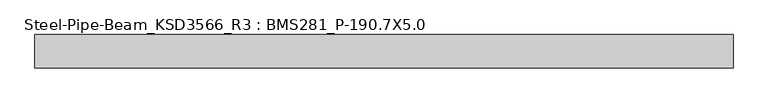
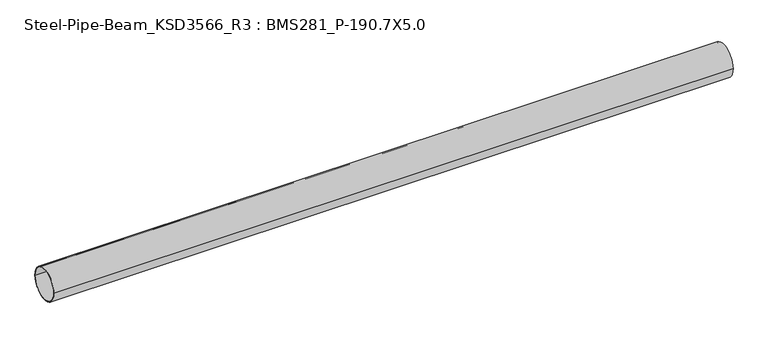
"""IFC4 building model written with IfcOpenShell, lengths in millimetres: member geometry, Steel-Pipe-Beam_KSD3566_R3 : BMS281_P-190.7X5.0."""

import ifcopenshell
import ifcopenshell.guid

model = None  # the IFC model being written
_history = None  # IfcOwnerHistory: only IFC2X3 demands one
_inside = {}  # id of a spatial element -> (the spatial element, [elements in it])
_under = {}  # id of a project, library or spatial element -> (it, [spatial elements below it])
_declared = {}  # id of a project -> (the project, [libraries it declares])
_typed = {}  # id of a type object -> (the type object, [elements of that type])
_made_of = {}  # id of a material, layer set ... -> (it, [elements and type objects made of it])


def new_model(schema):
    """Start an empty IFC model of exactly this schema.

    Asked for "IFC4X3", IfcOpenShell would pick the latest addendum, in which some entities
    have other attributes; the version numbers below select the first issue.
    IFC2X3 requires an IfcOwnerHistory on every rooted entity: one is made here for all.
    """
    global model, _history
    if schema == "IFC4X3":
        model = ifcopenshell.file(schema_version=(4, 3, 0, 0))
    else:
        model = ifcopenshell.file(schema=schema)
    _inside.clear()
    _under.clear()
    _declared.clear()
    _typed.clear()
    _made_of.clear()
    _history = None
    if model.schema == "IFC2X3":
        org = make("IfcOrganization", Name="unknown")
        user = make(
            "IfcPersonAndOrganization",
            ThePerson=make("IfcPerson", FamilyName="unknown"),
            TheOrganization=org,
        )
        app = make(
            "IfcApplication",
            ApplicationDeveloper=org,
            Version="unknown",
            ApplicationFullName="unknown",
            ApplicationIdentifier="unknown",
        )
        _history = make(
            "IfcOwnerHistory",
            OwningUser=user,
            OwningApplication=app,
            ChangeAction="ADDED",
            CreationDate=0,
        )
    return model


def make(cls, **values):
    """One entity of the class cls with the attributes given. An attribute that is None is left unset."""
    return model.create_entity(
        cls, **{name: value for name, value in values.items() if value is not None}
    )


def rooted(cls, **values):
    """An entity with a GlobalId (a new one), such as an element, a storey or a relation."""
    return make(cls, GlobalId=ifcopenshell.guid.new(), OwnerHistory=_history, **values)


def si_unit(unit_type, name, prefix=None):
    """IfcSIUnit, for example si_unit("LENGTHUNIT", "METRE", prefix="MILLI")."""
    return make("IfcSIUnit", UnitType=unit_type, Prefix=prefix, Name=name)


def assignment(units):
    """IfcUnitAssignment: the units of a project."""
    return None if units is None else make("IfcUnitAssignment", Units=units)


def point(xyz):
    """IfcCartesianPoint."""
    return None if xyz is None else make("IfcCartesianPoint", Coordinates=xyz)


def direction(xyz):
    """IfcDirection."""
    return None if xyz is None else make("IfcDirection", DirectionRatios=xyz)


def frame(location, z_axis=None, x_axis=None):
    """IfcAxis2Placement3D, a coordinate frame: its origin and axes. An axis left out is left unset."""
    return make(
        "IfcAxis2Placement3D",
        Location=point(location),
        Axis=direction(z_axis),
        RefDirection=direction(x_axis),
    )


def frame_2d(location, x_axis=None):
    """IfcAxis2Placement2D, a coordinate frame in the plane: its origin and x axis."""
    return make(
        "IfcAxis2Placement2D", Location=point(location), RefDirection=direction(x_axis)
    )


def origin():
    """The frame at (0, 0, 0) with its axes left unset."""
    return frame((0.0, 0.0, 0.0))


def origin_2d():
    """The frame at (0, 0) in the plane with its x axis left unset."""
    return frame_2d((0.0, 0.0))


def place(relative_to, where):
    """IfcLocalPlacement: puts the frame where relative to a parent placement (None: the world)."""
    return make(
        "IfcLocalPlacement", PlacementRelTo=relative_to, RelativePlacement=where
    )


def context(
    kind, dimensions, precision=None, world=None, true_north=None, identifier=None
):
    """IfcGeometricRepresentationContext, for example the 3D "Model" context."""
    return make(
        "IfcGeometricRepresentationContext",
        ContextIdentifier=identifier,
        ContextType=kind,
        CoordinateSpaceDimension=dimensions,
        Precision=precision,
        WorldCoordinateSystem=world,
        TrueNorth=true_north,
    )


def project(units=None, contexts=None):
    """IfcProject with its units and contexts."""
    return rooted(
        "IfcProject",
        Name="project",
        RepresentationContexts=contexts,
        UnitsInContext=assignment(units),
    )


def spatial(cls, under=None, at=None, **own):
    """A site, building, storey or space (cls), placed at a placement, below another one or the project."""
    s = rooted(cls, ObjectPlacement=at, **own)
    if under is not None:
        _under.setdefault(under.id(), (under, []))[1].append(s)
    return s


def circle_curve(where, radius):
    """IfcCircle in the frame where."""
    return make("IfcCircle", Position=where, Radius=radius)


def trimmed(basis, trim1, trim2, sense, master):
    """IfcTrimmedCurve: the piece of a basis curve between two trims."""
    return make(
        "IfcTrimmedCurve",
        BasisCurve=basis,
        Trim1=trim1,
        Trim2=trim2,
        SenseAgreement=sense,
        MasterRepresentation=master,
    )


def segment(curve, same_sense, transition):
    """IfcCompositeCurveSegment."""
    return make(
        "IfcCompositeCurveSegment",
        Transition=transition,
        SameSense=same_sense,
        ParentCurve=curve,
    )


def composite_curve(segments, self_intersect=None):
    """IfcCompositeCurve: segments joined end to end."""
    return make("IfcCompositeCurve", Segments=segments, SelfIntersect=self_intersect)


def outline(outer, holes=None, kind="AREA"):
    """IfcArbitraryClosedProfileDef: a profile drawn as a closed curve; with holes, ...WithVoids."""
    if holes is None:
        return make("IfcArbitraryClosedProfileDef", ProfileType=kind, OuterCurve=outer)
    return make(
        "IfcArbitraryProfileDefWithVoids",
        ProfileType=kind,
        OuterCurve=outer,
        InnerCurves=holes,
    )


def extrude(swept, where, along, depth):
    """IfcExtrudedAreaSolid: the profile swept, set in the frame where, extruded along a direction by depth."""
    return make(
        "IfcExtrudedAreaSolid",
        SweptArea=swept,
        Position=where,
        ExtrudedDirection=direction(along),
        Depth=depth,
    )


def shape(context_of_items, identifier, shape_type, items):
    """IfcShapeRepresentation: the items that make up one representation, for example the "Body"."""
    return make(
        "IfcShapeRepresentation",
        ContextOfItems=context_of_items,
        RepresentationIdentifier=identifier,
        RepresentationType=shape_type,
        Items=items,
    )


def source(mapping_origin, context_of_items, identifier, shape_type, items):
    """IfcRepresentationMap: a shape defined once, which mapped items show again and again."""
    return make(
        "IfcRepresentationMap",
        MappingOrigin=mapping_origin,
        MappedRepresentation=shape(context_of_items, identifier, shape_type, items),
    )


def transform(
    local_origin,
    x_axis=None,
    y_axis=None,
    z_axis=None,
    scale=None,
    scale2=None,
    scale3=None,
    uniform=True,
):
    """IfcCartesianTransformationOperator3D, or its non-uniform kind. x_axis, y_axis, z_axis: its Axis1, 2, 3."""
    if uniform:
        return make(
            "IfcCartesianTransformationOperator3D",
            Axis1=direction(x_axis),
            Axis2=direction(y_axis),
            LocalOrigin=point(local_origin),
            Scale=scale,
            Axis3=direction(z_axis),
        )
    return make(
        "IfcCartesianTransformationOperator3DnonUniform",
        Axis1=direction(x_axis),
        Axis2=direction(y_axis),
        LocalOrigin=point(local_origin),
        Scale=scale,
        Axis3=direction(z_axis),
        Scale2=scale2,
        Scale3=scale3,
    )


def mapped(mapping_source, mapping_target):
    """IfcMappedItem: shows the shape of a source again, moved by a transform."""
    return make(
        "IfcMappedItem", MappingSource=mapping_source, MappingTarget=mapping_target
    )


def made_of(thing, what):
    """Note that an element or type object is made of a material, layer set ...; save() writes the relation."""
    if what is not None:
        _made_of.setdefault(what.id(), (what, []))[1].append(thing)
    return thing


def element(
    cls,
    number,
    at=None,
    inside=None,
    cuts=None,
    type_object=None,
    material=None,
    context=None,
    identifier="Body",
    shape_type=None,
    held_by="IfcProductDefinitionShape",
    body=None,
    shapes=None,
    **own,
):
    """One element of the class cls, such as IfcWall. Its Tag is "e" and its number.

    at: its placement. inside: the storey or other place that contains it. cuts: it is an
    opening in that element (IfcRelVoidsElement). A single representation is given by context,
    identifier, shape_type and body (its items); several are given by shapes. held_by: the class
    of the entity that holds the representations. save() writes the other relations.
    """
    e = rooted(cls, Tag="e%d" % number, ObjectPlacement=at, **own)
    if body is not None:
        shapes = [shape(context, identifier, shape_type, body)]
    if shapes is not None:
        e.Representation = make(held_by, Representations=shapes)
    if inside is not None:
        _inside.setdefault(inside.id(), (inside, []))[1].append(e)
    if cuts is not None:
        rooted(
            "IfcRelVoidsElement", RelatingBuildingElement=cuts, RelatedOpeningElement=e
        )
    if type_object is not None:
        _typed.setdefault(type_object.id(), (type_object, []))[1].append(e)
    return made_of(e, material)


def aggregate(whole, parts):
    """IfcRelAggregates: a whole, such as a stair, and the parts it consists of."""
    return rooted("IfcRelAggregates", RelatingObject=whole, RelatedObjects=parts)


def save(model, path):
    """Write the relations noted so far, then the file.

    IfcRelAggregates (storeys below a building ...), IfcRelContainedInSpatialStructure (elements
    in a storey), IfcRelDefinesByType, IfcRelAssociatesMaterial and IfcRelDeclares: one each for
    every whole, place, type object, material and project.
    """
    for whole, parts in _under.values():
        aggregate(whole, parts)
    for where, things in _inside.values():
        rooted(
            "IfcRelContainedInSpatialStructure",
            RelatedElements=things,
            RelatingStructure=where,
        )
    for kind, things in _typed.values():
        rooted("IfcRelDefinesByType", RelatedObjects=things, RelatingType=kind)
    for what, things in _made_of.values():
        rooted("IfcRelAssociatesMaterial", RelatedObjects=things, RelatingMaterial=what)
    for by, libraries in _declared.values():
        rooted("IfcRelDeclares", RelatingContext=by, RelatedDefinitions=libraries)
    model.write(path)


def steel_pipe_beam_ksd3566_r3_bms281_p_190_7x5_0_885972b8(model_context):
    return source(origin(), model_context, "Body", "SweptSolid", [
        extrude(outline(composite_curve([segment(trimmed(circle_curve(origin_2d(), 95.35), [point((-95.35, 0.0))], [point((95.35, 0.0))], False, "CARTESIAN"), True, "CONTINUOUS"), segment(trimmed(circle_curve(origin_2d(), 95.35), [point((95.35, 0.0))], [point((-95.35, 0.0))], False, "CARTESIAN"), True, "CONTINUOUS")], self_intersect=False), holes=[composite_curve([segment(trimmed(circle_curve(origin_2d(), 90.35), [point((90.35, 0.0))], [point((-90.35, 0.0))], True, "CARTESIAN"), True, "CONTINUOUS"), segment(trimmed(circle_curve(origin_2d(), 90.35), [point((-90.35, 0.0))], [point((90.35, 0.0))], True, "CARTESIAN"), True, "CONTINUOUS")], self_intersect=False)]), frame((-1965.4784034, 0.0, 0.0), z_axis=(1.0, 0.0, 0.0), x_axis=(0.0, 1.0, 0.0)), (0.0, 0.0, 1.0), 3968.5849078),
    ])


if __name__ == "__main__":
    model = new_model("IFC4")
    model_context = context("Model", 3, world=origin())
    ifc_project = project(units=[si_unit("LENGTHUNIT", "METRE", prefix="MILLI")], contexts=[model_context])
    site = spatial("IfcSite", under=ifc_project)
    building = spatial("IfcBuilding", under=site)
    placement = place(None, origin())
    steel_pipe_beam_ksd3566_r3_bms281_p_190_7x5_0_shape = steel_pipe_beam_ksd3566_r3_bms281_p_190_7x5_0_885972b8(model_context)
    element("IfcMember", 1, ObjectType="Steel-Pipe-Beam_KSD3566_R3 : BMS281_P-190.7X5.0", at=placement, inside=building, context=model_context, shape_type="MappedRepresentation", body=[
        mapped(steel_pipe_beam_ksd3566_r3_bms281_p_190_7x5_0_shape, transform((0.0, 0.0, 0.0), x_axis=(1.0, 0.0, 0.0), y_axis=(0.0, 1.0, 0.0), z_axis=(0.0, 0.0, 1.0))),
    ])
    save(model, "model.ifc")

# Revit data of these elements
# Type "Steel-Pipe-Beam_KSD3566_R3 : BMS281_P-190.7X5.0"
#   Keynote = "P-190.7X5.0"
#   SteelWeight = "Light"
#   t = 0.0050 m
#   Surface Area = 0.599102 m²/m
#   Section Area = 29.1697 cm²
#   Mass per Unit Length = 22.8982 kg/m
#   Length [instance default] = 1.5000 m
#   D = 0.1907 m
#   hec_material4 [instance default] = none
#   hec_material3 [instance default] = none
#   hec_material2 [instance default] = none
#   hec_material1 [instance default] = none
#   Structural Material [instance default] = Steel, 45-345
#   Assembly Code = ""
# Element 1 (IfcMember, "Steel-Pipe-Beam_KSD3566_R3 : BMS281_P-190.7X5.0")
#   Structural Material = none
# Materials
#   "Steel, 45-345": class "Metal", colour RGB 189 187 185, transparency 0, Description = "Steel 345 MPa", Cost = 0
